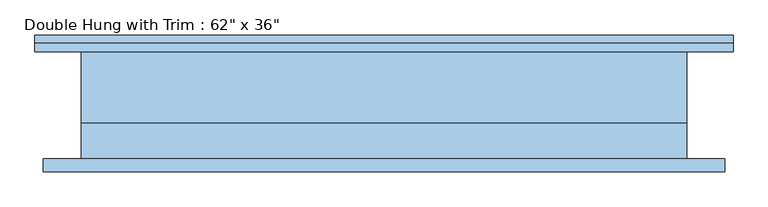
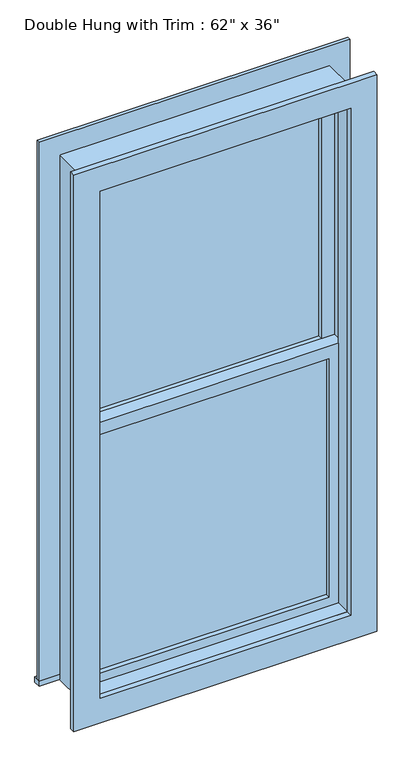
"""IFC4 building model written with IfcOpenShell, lengths in millimetres: window geometry."""

import ifcopenshell
import ifcopenshell.guid

model = None  # the IFC model being written
_history = None  # IfcOwnerHistory: only IFC2X3 demands one
_inside = {}  # id of a spatial element -> (the spatial element, [elements in it])
_under = {}  # id of a project, library or spatial element -> (it, [spatial elements below it])
_declared = {}  # id of a project -> (the project, [libraries it declares])
_typed = {}  # id of a type object -> (the type object, [elements of that type])
_made_of = {}  # id of a material, layer set ... -> (it, [elements and type objects made of it])


def new_model(schema):
    """Start an empty IFC model of exactly this schema.

    Asked for "IFC4X3", IfcOpenShell would pick the latest addendum, in which some entities
    have other attributes; the version numbers below select the first issue.
    IFC2X3 requires an IfcOwnerHistory on every rooted entity: one is made here for all.
    """
    global model, _history
    if schema == "IFC4X3":
        model = ifcopenshell.file(schema_version=(4, 3, 0, 0))
    else:
        model = ifcopenshell.file(schema=schema)
    _inside.clear()
    _under.clear()
    _declared.clear()
    _typed.clear()
    _made_of.clear()
    _history = None
    if model.schema == "IFC2X3":
        org = make("IfcOrganization", Name="unknown")
        user = make(
            "IfcPersonAndOrganization",
            ThePerson=make("IfcPerson", FamilyName="unknown"),
            TheOrganization=org,
        )
        app = make(
            "IfcApplication",
            ApplicationDeveloper=org,
            Version="unknown",
            ApplicationFullName="unknown",
            ApplicationIdentifier="unknown",
        )
        _history = make(
            "IfcOwnerHistory",
            OwningUser=user,
            OwningApplication=app,
            ChangeAction="ADDED",
            CreationDate=0,
        )
    return model


def make(cls, **values):
    """One entity of the class cls with the attributes given. An attribute that is None is left unset."""
    return model.create_entity(
        cls, **{name: value for name, value in values.items() if value is not None}
    )


def rooted(cls, **values):
    """An entity with a GlobalId (a new one), such as an element, a storey or a relation."""
    return make(cls, GlobalId=ifcopenshell.guid.new(), OwnerHistory=_history, **values)


def si_unit(unit_type, name, prefix=None):
    """IfcSIUnit, for example si_unit("LENGTHUNIT", "METRE", prefix="MILLI")."""
    return make("IfcSIUnit", UnitType=unit_type, Prefix=prefix, Name=name)


def assignment(units):
    """IfcUnitAssignment: the units of a project."""
    return None if units is None else make("IfcUnitAssignment", Units=units)


def point(xyz):
    """IfcCartesianPoint."""
    return None if xyz is None else make("IfcCartesianPoint", Coordinates=xyz)


def direction(xyz):
    """IfcDirection."""
    return None if xyz is None else make("IfcDirection", DirectionRatios=xyz)


def frame(location, z_axis=None, x_axis=None):
    """IfcAxis2Placement3D, a coordinate frame: its origin and axes. An axis left out is left unset."""
    return make(
        "IfcAxis2Placement3D",
        Location=point(location),
        Axis=direction(z_axis),
        RefDirection=direction(x_axis),
    )


def origin():
    """The frame at (0, 0, 0) with its axes left unset."""
    return frame((0.0, 0.0, 0.0))


def place(relative_to, where):
    """IfcLocalPlacement: puts the frame where relative to a parent placement (None: the world)."""
    return make(
        "IfcLocalPlacement", PlacementRelTo=relative_to, RelativePlacement=where
    )


def context(
    kind, dimensions, precision=None, world=None, true_north=None, identifier=None
):
    """IfcGeometricRepresentationContext, for example the 3D "Model" context."""
    return make(
        "IfcGeometricRepresentationContext",
        ContextIdentifier=identifier,
        ContextType=kind,
        CoordinateSpaceDimension=dimensions,
        Precision=precision,
        WorldCoordinateSystem=world,
        TrueNorth=true_north,
    )


def project(units=None, contexts=None):
    """IfcProject with its units and contexts."""
    return rooted(
        "IfcProject",
        Name="project",
        RepresentationContexts=contexts,
        UnitsInContext=assignment(units),
    )


def spatial(cls, under=None, at=None, **own):
    """A site, building, storey or space (cls), placed at a placement, below another one or the project."""
    s = rooted(cls, ObjectPlacement=at, **own)
    if under is not None:
        _under.setdefault(under.id(), (under, []))[1].append(s)
    return s


def polyline(points):
    """IfcPolyline through the points."""
    return make("IfcPolyline", Points=[point(p) for p in points])


def outline(outer, holes=None, kind="AREA"):
    """IfcArbitraryClosedProfileDef: a profile drawn as a closed curve; with holes, ...WithVoids."""
    if holes is None:
        return make("IfcArbitraryClosedProfileDef", ProfileType=kind, OuterCurve=outer)
    return make(
        "IfcArbitraryProfileDefWithVoids",
        ProfileType=kind,
        OuterCurve=outer,
        InnerCurves=holes,
    )


def extrude(swept, where, along, depth):
    """IfcExtrudedAreaSolid: the profile swept, set in the frame where, extruded along a direction by depth."""
    return make(
        "IfcExtrudedAreaSolid",
        SweptArea=swept,
        Position=where,
        ExtrudedDirection=direction(along),
        Depth=depth,
    )


def shape(context_of_items, identifier, shape_type, items):
    """IfcShapeRepresentation: the items that make up one representation, for example the "Body"."""
    return make(
        "IfcShapeRepresentation",
        ContextOfItems=context_of_items,
        RepresentationIdentifier=identifier,
        RepresentationType=shape_type,
        Items=items,
    )


def source(mapping_origin, context_of_items, identifier, shape_type, items):
    """IfcRepresentationMap: a shape defined once, which mapped items show again and again."""
    return make(
        "IfcRepresentationMap",
        MappingOrigin=mapping_origin,
        MappedRepresentation=shape(context_of_items, identifier, shape_type, items),
    )


def transform(
    local_origin,
    x_axis=None,
    y_axis=None,
    z_axis=None,
    scale=None,
    scale2=None,
    scale3=None,
    uniform=True,
):
    """IfcCartesianTransformationOperator3D, or its non-uniform kind. x_axis, y_axis, z_axis: its Axis1, 2, 3."""
    if uniform:
        return make(
            "IfcCartesianTransformationOperator3D",
            Axis1=direction(x_axis),
            Axis2=direction(y_axis),
            LocalOrigin=point(local_origin),
            Scale=scale,
            Axis3=direction(z_axis),
        )
    return make(
        "IfcCartesianTransformationOperator3DnonUniform",
        Axis1=direction(x_axis),
        Axis2=direction(y_axis),
        LocalOrigin=point(local_origin),
        Scale=scale,
        Axis3=direction(z_axis),
        Scale2=scale2,
        Scale3=scale3,
    )


def mapped(mapping_source, mapping_target):
    """IfcMappedItem: shows the shape of a source again, moved by a transform."""
    return make(
        "IfcMappedItem", MappingSource=mapping_source, MappingTarget=mapping_target
    )


def made_of(thing, what):
    """Note that an element or type object is made of a material, layer set ...; save() writes the relation."""
    if what is not None:
        _made_of.setdefault(what.id(), (what, []))[1].append(thing)
    return thing


def element(
    cls,
    number,
    at=None,
    inside=None,
    cuts=None,
    type_object=None,
    material=None,
    context=None,
    identifier="Body",
    shape_type=None,
    held_by="IfcProductDefinitionShape",
    body=None,
    shapes=None,
    **own,
):
    """One element of the class cls, such as IfcWall. Its Tag is "e" and its number.

    at: its placement. inside: the storey or other place that contains it. cuts: it is an
    opening in that element (IfcRelVoidsElement). A single representation is given by context,
    identifier, shape_type and body (its items); several are given by shapes. held_by: the class
    of the entity that holds the representations. save() writes the other relations.
    """
    e = rooted(cls, Tag="e%d" % number, ObjectPlacement=at, **own)
    if body is not None:
        shapes = [shape(context, identifier, shape_type, body)]
    if shapes is not None:
        e.Representation = make(held_by, Representations=shapes)
    if inside is not None:
        _inside.setdefault(inside.id(), (inside, []))[1].append(e)
    if cuts is not None:
        rooted(
            "IfcRelVoidsElement", RelatingBuildingElement=cuts, RelatedOpeningElement=e
        )
    if type_object is not None:
        _typed.setdefault(type_object.id(), (type_object, []))[1].append(e)
    return made_of(e, material)


def aggregate(whole, parts):
    """IfcRelAggregates: a whole, such as a stair, and the parts it consists of."""
    return rooted("IfcRelAggregates", RelatingObject=whole, RelatedObjects=parts)


def save(model, path):
    """Write the relations noted so far, then the file.

    IfcRelAggregates (storeys below a building ...), IfcRelContainedInSpatialStructure (elements
    in a storey), IfcRelDefinesByType, IfcRelAssociatesMaterial and IfcRelDeclares: one each for
    every whole, place, type object, material and project.
    """
    for whole, parts in _under.values():
        aggregate(whole, parts)
    for where, things in _inside.values():
        rooted(
            "IfcRelContainedInSpatialStructure",
            RelatedElements=things,
            RelatingStructure=where,
        )
    for kind, things in _typed.values():
        rooted("IfcRelDefinesByType", RelatedObjects=things, RelatingType=kind)
    for what, things in _made_of.values():
        rooted("IfcRelAssociatesMaterial", RelatedObjects=things, RelatingMaterial=what)
    for by, libraries in _declared.values():
        rooted("IfcRelDeclares", RelatingContext=by, RelatedDefinitions=libraries)
    model.write(path)


def window_f7e5e0d9(model_context):
    return source(origin(), model_context, "Body", "SweptSolid", [
        extrude(outline(polyline([(-393.7, 1.5875), (393.7, 1.5875), (393.7, -11.1125), (-393.7, -11.1125), (-393.7, 1.5875)])), frame((0.0, 0.0, 571.5), z_axis=(0.0, 0.0, 1.0), x_axis=(1.0, 0.0, 0.0)), (0.0, 0.0, 1.0), 854.075),
        extrude(outline(polyline([(1470.025, -438.15), (527.05, -438.15), (527.05, 438.15), (1470.025, 438.15), (1470.025, -438.15)]), holes=[polyline([(1425.575, -393.7), (1425.575, 393.7), (571.5, 393.7), (571.5, -393.7), (1425.575, -393.7)])]), frame((0.0, -26.9875, 0.0), z_axis=(0.0, 1.0, 0.0), x_axis=(0.0, 0.0, 1.0)), (0.0, 0.0, 1.0), 44.45),
        extrude(outline(polyline([(-527.05, 106.3625), (527.05, 106.3625), (527.05, 80.9625), (-527.05, 80.9625), (-527.05, 106.3625)])), frame((0.0, 0.0, 508.0), z_axis=(0.0, 0.0, 1.0), x_axis=(1.0, 0.0, 0.0)), (0.0, 0.0, 1.0), 19.05),
        extrude(outline(polyline([(2368.55, -438.15), (2368.55, 438.15), (527.05, 438.15), (527.05, 527.05), (2457.45, 527.05), (2457.45, -527.05), (527.05, -527.05), (527.05, -438.15), (2368.55, -438.15)])), frame((0.0, 80.9625, 0.0), z_axis=(0.0, 1.0, 0.0), x_axis=(0.0, 0.0, 1.0)), (0.0, 0.0, 1.0), 12.7),
        extrude(outline(polyline([(2444.75, 514.35), (2444.75, -514.35), (450.85, -514.35), (450.85, 514.35), (2444.75, 514.35)]), holes=[polyline([(2355.85, 425.45), (539.75, 425.45), (539.75, -425.45), (2355.85, -425.45), (2355.85, 425.45)])]), frame((0.0, -100.0125, 0.0), z_axis=(0.0, 1.0, 0.0), x_axis=(0.0, 0.0, 1.0)), (0.0, 0.0, 1.0), 19.05),
        extrude(outline(polyline([(393.7, 33.3375), (-393.7, 33.3375), (-393.7, 46.0375), (393.7, 46.0375), (393.7, 33.3375)])), frame((0.0, 0.0, 1470.025), z_axis=(0.0, 0.0, 1.0), x_axis=(1.0, 0.0, 0.0)), (0.0, 0.0, 1.0), 854.075),
        extrude(outline(polyline([(2368.55, -438.15), (1425.575, -438.15), (1425.575, 438.15), (2368.55, 438.15), (2368.55, -438.15)]), holes=[polyline([(2324.1, -393.7), (2324.1, 393.7), (1470.025, 393.7), (1470.025, -393.7), (2324.1, -393.7)])]), frame((0.0, 17.4625, 0.0), z_axis=(0.0, 1.0, 0.0), x_axis=(0.0, 0.0, 1.0)), (0.0, 0.0, 1.0), 44.45),
        extrude(outline(polyline([(2387.6, -457.2), (508.0, -457.2), (508.0, 457.2), (2387.6, 457.2), (2387.6, -457.2)]), holes=[polyline([(2355.85, -425.45), (2355.85, 425.45), (539.75, 425.45), (539.75, -425.45), (2355.85, -425.45)])]), frame((0.0, -80.9625, 0.0), z_axis=(0.0, 1.0, 0.0), x_axis=(0.0, 0.0, 1.0)), (0.0, 0.0, 1.0), 53.975),
        extrude(outline(polyline([(2387.6, 457.2), (2387.6, -457.2), (508.0, -457.2), (508.0, 457.2), (2387.6, 457.2)]), holes=[polyline([(2368.55, 438.15), (527.05, 438.15), (527.05, -438.15), (2368.55, -438.15), (2368.55, 438.15)])]), frame((0.0, -26.9875, 0.0), z_axis=(0.0, 1.0, 0.0), x_axis=(0.0, 0.0, 1.0)), (0.0, 0.0, 1.0), 107.95),
    ])


if __name__ == "__main__":
    model = new_model("IFC4")
    model_context = context("Model", 3, world=origin())
    ifc_project = project(units=[si_unit("LENGTHUNIT", "METRE", prefix="MILLI")], contexts=[model_context])
    site = spatial("IfcSite", under=ifc_project)
    building = spatial("IfcBuilding", under=site)
    placement = place(None, origin())
    window_shape = window_f7e5e0d9(model_context)
    element("IfcWindow", 1, ObjectType="Double Hung with Trim : 62\" x 36\"", at=placement, inside=building, context=model_context, shape_type="MappedRepresentation", body=[
        mapped(window_shape, transform((0.0, 0.0, 0.0), x_axis=(1.0, 0.0, 0.0), y_axis=(0.0, 1.0, 0.0), z_axis=(0.0, 0.0, 1.0))),
    ])
    save(model, "model.ifc")

# Revit data of these elements
# Type "Double Hung with Trim : 62\" x 36\""
#   Type Mark = "65"
#   COBie.Type.CreatedBy = "doug.wood@us.ibm.com"
#   COBie.Type.CreatedOn = "2016-04-14T02:07:26"
#   COBie.Type.Name = "Windows_Double Hung with Trim_62\" x 36\"_65"
#   COBie.Type.Category = "23-30 20 17 17 14 : Double-Hung Windows"
#   COBie.Type.Description = "Double Hung with Trim_62\" x 36\""
#   COBie.Type.Manufacturer = ""
#   COBie.Type.ModelNumber = ""
#   Construction Type Id = "GSP4R"
#   Assembly Code = "B2020100"
#   Analytic Construction = "1/8 in Pilkington single glazing"
#   COBie.Type.ReplacementCost = 0
#   Visual Light Transmittance = 0.9
#   Solar Heat Gain Coefficient = 0.78
#   Heat Transfer Coefficient (U) = 3.6886 W/(m²·K)
#   Height = 6' - 2"
#   Default Sill Height = 1' - 8"
#   Trim Projection - Ext. = 0' - 0 1/2"
#   Trim Projection - Int. = 0' - 0 3/4"
#   Trim Width - Exterior = 0' - 3 1/2"
#   Trim Width - Interior = 0' - 3 1/2"
#   Width = 3' - 0"
#   Window Inset = 0' - 0 3/4"
#   COBie.Type = no
#   Glass Pane Material = Glass
#   Sash Material = Sash - White
#   Trim Exterior Material = Trim - White
#   Trim Interior Material = Trim - White
#   Wall Closure = (empty or 0)
# Element 1 (IfcWindow, "Double Hung with Trim : 62\" x 36\"")
#   Materials on its faces: "Sash - White", "Trim - White", "Glass"
# Materials
#   "Glass": class "Glass", colour RGB 0 128 192, transparency 0.75, Description = "Soda Lime Glass", Cost = 0
#   "Sash - White": class "Wood", colour RGB 255 255 255, transparency 0, Cost = 0
#   "Trim - White": class "Wood", colour RGB 255 255 255, transparency 0, Cost = 0
